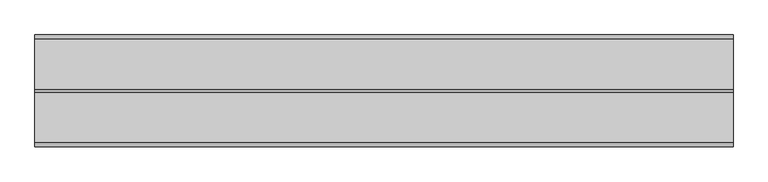
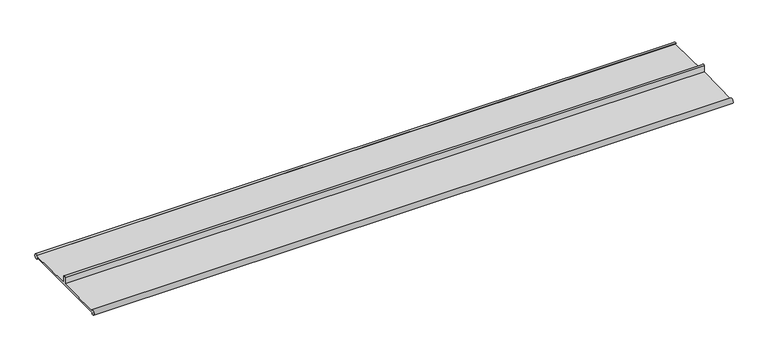
"""IFC4 building model written with IfcOpenShell, lengths in millimetres: proxy geometry, TN_ПВХ_ТПО_Гидрошпонка ТехноНИКОЛЬ : ПВХ Гидрошпонка ТехноНИКОЛЬ IC-240-2."""

from ifc_helpers import new_model, si_unit, point, frame, frame_2d, origin, place, context, project, spatial, polyline, circle_curve, trimmed, segment, composite_curve, outline, extrude, source, transform, mapped, element, save


def specialty_equipment_ccce3da2(model_context):
    return source(origin(), model_context, "Body", "SweptSolid", [
        extrude(outline(composite_curve([segment(polyline([(115.0007615, 0.0), (-115.0007615, 0.0), (-111.4652276, -3.5355339)]), True, "CONTINUOUS"), segment(trimmed(circle_curve(frame_2d((-114.3714227, 1.518146)), 5.8297212), [point((-111.4652276, -3.5355339))], [point((-111.4652276, 6.5718258))], False, "CARTESIAN"), True, "CONTINUOUS"), segment(polyline([(-111.4652276, 6.5718258), (-115.0007615, 3.0362919), (-2.5, 5.0), (-2.5, 20.0)]), True, "CONTINUOUS"), segment(trimmed(circle_curve(frame_2d((0.0, 20.0)), 2.5), [point((-2.5, 20.0))], [point((2.5, 20.0))], False, "CARTESIAN"), True, "CONTINUOUS"), segment(polyline([(2.5, 20.0), (2.5, 5.0), (115.0007615, 3.0362919), (111.4652276, 6.5718258)]), True, "CONTINUOUS"), segment(trimmed(circle_curve(frame_2d((114.3714227, 1.518146)), 5.8297212), [point((111.4652276, 6.5718258))], [point((111.4652276, -3.5355339))], False, "CARTESIAN"), True, "CONTINUOUS"), segment(polyline([(111.4652276, -3.5355339), (115.0007615, 0.0)]), True, "CONTINUOUS")], self_intersect=False)), frame((0.0, 0.0, 0.0), z_axis=(1.0, 0.0, 0.0), x_axis=(0.0, 1.0, 0.0)), (0.0, 0.0, 1.0), 1500.0),
    ])


if __name__ == "__main__":
    model = new_model("IFC4")
    model_context = context("Model", 3, world=origin())
    ifc_project = project(units=[si_unit("LENGTHUNIT", "METRE", prefix="MILLI")], contexts=[model_context])
    site = spatial("IfcSite", under=ifc_project)
    building = spatial("IfcBuilding", under=site)
    placement = place(None, origin())
    specialty_equipment_shape = specialty_equipment_ccce3da2(model_context)
    element("IfcBuildingElementProxy", 1, Name="TN_ПВХ_ТПО_Гидрошпонка ТехноНИКОЛЬ : ПВХ Гидрошпонка ТехноНИКОЛЬ IC-240-2", ObjectType="TN_ПВХ_ТПО_Гидрошпонка ТехноНИКОЛЬ : ПВХ Гидрошпонка ТехноНИКОЛЬ IC-240-2", at=placement, inside=building, context=model_context, shape_type="MappedRepresentation", body=[
        mapped(specialty_equipment_shape, transform((0.0, 0.0, 0.0), x_axis=(1.0, 0.0, 0.0), y_axis=(0.0, 1.0, 0.0), z_axis=(0.0, 0.0, 1.0))),
    ])
    save(model, "model.ifc")

# Revit data of these elements
# Type "TN_ПВХ_ТПО_Гидрошпонка ТехноНИКОЛЬ : ПВХ Гидрошпонка ТехноНИКОЛЬ IC-240-2"
#   Description = "Внутренняя гидрошпонка для герметизации рабочих швов бетонирования в монолитных конструкциях при новом строительстве - подземных частей зданий, подземных парковок, тоннелей, коллекторов, дамб, каналов, резервуаров, бассейнов, очистных сооружений и пр."
#   Type Comments = "п.м."
#   Manufacturer = "ТехноНИКОЛЬ"
#   URL = "https://www.tn.ru/catalogue/dopolnitelnye_element2/gidroizoljacionnaja_shponka_tipa_vr_220/"
#   ADSK_Примечание = ""
#   ADSK_Обозначение [instance default] = "ТехноНИКОЛЬ"
#   ADSK_Наименование = "ПВХ Гидрошпонка ТехноНИКОЛЬ IC-240-2, 20м/рул"
#   ADSK_Масса_Текст = ""
#   ADSK_Марка = ""
#   ADSK_Код изделия = "499885"
#   ADSK_Завод-изготовитель [instance default] = "ТехноНИКОЛЬ"
#   ADSK_Единица измерения [instance default] = "п.м."
#   ADSK_Группирование = "Гидрошпонки"
#   ADSK_URL страницы изделия = "https://www.tn.ru/catalogue/dopolnitelnye_element2/gidroizoljacionnaja_shponka_tipa_vr_220/"
#   ADSK_URL документации изделия = "https://nav.tn.ru/upload/iblock/67f/Katalog-i-rekomendatsii-po-primeneniyu_Gidroshponki-TEKHNONIKOL.PDF"
#   built-in parameter 1001306 [instance default] = 3.28084 (stored number, unit not read)
#   ADSK_Размер_Длина [instance default] = 1000 mm
#   ADSK_Количество [instance default] = 1
#   ПВХ_ТПО Гидрошпонка ТехноНИКОЛЬ EC-320-4 = no
#   ПВХ Гидрошпонка ТехноНИКОЛЬ IM-260/50 = no
#   ПВХ Гидрошпонка ТехноНИКОЛЬ IM-240/20 = no
#   ПВХ Гидрошпонка ТехноНИКОЛЬ IC-240-6 = no
#   ПВХ Гидрошпонка ТехноНИКОЛЬ IC-125-2SP = no
#   ПВХ Гидрошпонка ТехноНИКОЛЬ EM-260/50 = no
#   ПВХ Гидрошпонка ТехноНИКОЛЬ EM-260/20 = no
#   ПВХ Гидрошпонка ТехноНИКОЛЬ EC-320-4 = no
#   ПВХ Гидрошпонка ТехноНИКОЛЬ EC-220-3 = no
#   ПВХ_ТПО Гидрошпонка ТехноНИКОЛЬ EC-220-3 = no
#   ПВХ Гидрошпонка ТехноНИКОЛЬ IC-240-2 = yes
#   Материал = TN_ПВХ_Черный
#   Default Elevation = 0
# Element 1 (IfcBuildingElementProxy, "TN_ПВХ_ТПО_Гидрошпонка ТехноНИКОЛЬ : ПВХ Гидрошпонка ТехноНИКОЛЬ IC-240-2")
#   built-in parameter 1001306 = 4.92126 (stored number, unit not read)
#   ADSK_Размер_Длина = 1500 mm
#   ADSK_Количество = 1.5
#   Materials on its faces: "TN_ПВХ_Черный"
# Materials
#   "TN_ПВХ_Черный": class "Типовые", colour RGB 48 48 48, transparency 0, Cost = 0
